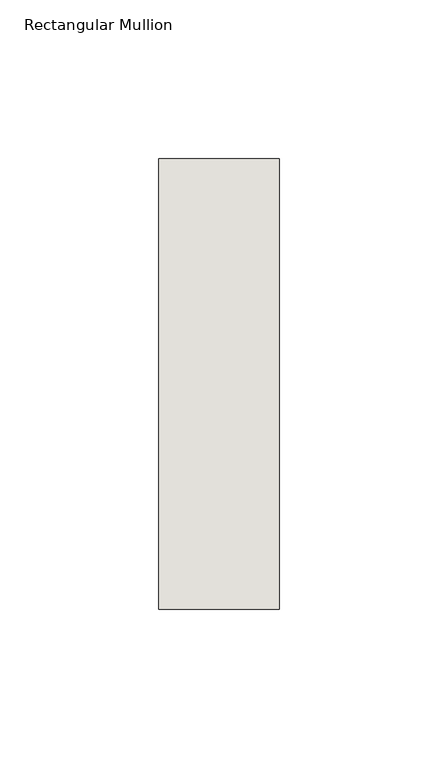
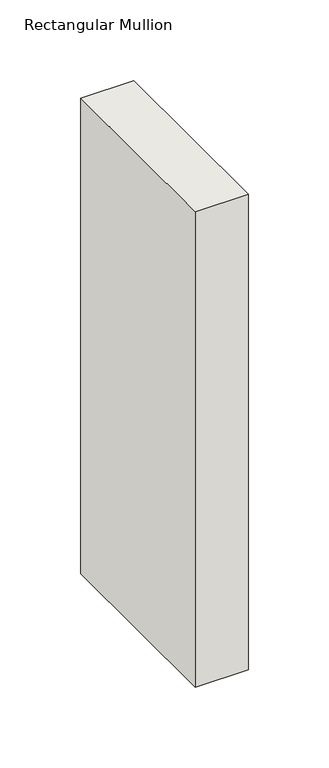
"""IFC4 building model written with IfcOpenShell, lengths in millimetres: wall geometry, Rectangular Mullion : NLRS_21_CWM_hsb-regel 38x142_gen_rsf."""

from ifc_helpers import new_model, si_unit, frame, origin, place, context, project, spatial, polyline, outline, extrude, source, transform, mapped, element, save


def rectangular_mullion_923ec213(model_context):
    return source(origin(), model_context, "Body", "SweptSolid", [
        extrude(outline(polyline([(0.0, -71.0), (-38.0, -71.0), (-38.0, 71.0), (0.0, 71.0), (0.0, -71.0)])), frame((0.0, 0.0, -359.9999997), z_axis=(0.0, 0.0, 1.0), x_axis=(1.0, 0.0, 0.0)), (0.0, 0.0, 1.0), 359.9999997),
    ])


if __name__ == "__main__":
    model = new_model("IFC4")
    model_context = context("Model", 3, world=origin())
    ifc_project = project(units=[si_unit("LENGTHUNIT", "METRE", prefix="MILLI")], contexts=[model_context])
    site = spatial("IfcSite", under=ifc_project)
    building = spatial("IfcBuilding", under=site)
    placement = place(None, origin())
    rectangular_mullion_shape = rectangular_mullion_923ec213(model_context)
    element("IfcWall", 1, ObjectType="Rectangular Mullion : NLRS_21_CWM_hsb-regel 38x142_gen_rsf", at=placement, inside=building, context=model_context, shape_type="MappedRepresentation", body=[
        mapped(rectangular_mullion_shape, transform((0.0, 0.0, 0.0), x_axis=(1.0, 0.0, 0.0), y_axis=(0.0, 1.0, 0.0), z_axis=(0.0, 0.0, 1.0))),
    ])
    save(model, "model.ifc")

# Revit data of these elements
# Type "Rectangular Mullion : NLRS_21_CWM_hsb-regel 38x142_gen_rsf"
#   Type IfcGUID = "07M7mRoiH1CR8m_RSKIwpF"
#   Assembly Code = "21.10"
#   IfcExportAs = "IfcWall"
#   built-in parameter 1007322 = 0.465879 (stored number, unit not read)
#   built-in parameter 1007321 = 0.062336 (stored number, unit not read)
#   built-in parameter 1007320 = 0.062336 (stored number, unit not read)
# Element 1 (IfcWall, "Rectangular Mullion : NLRS_21_CWM_hsb-regel 38x142_gen_rsf")
#   Materials on its faces: "NLRS_i2_hout naaldhout vuren_gen_rsf"
# Materials
#   "NLRS_i2_hout naaldhout vuren_gen_rsf": class "I - Hout", colour RGB 234 199 147, transparency 0, Keynote = "i2", Manufacturer = "Revit Standards Foundation", URL = "www.revitstandards.org", Description = "hout vuren", Cost = 0
